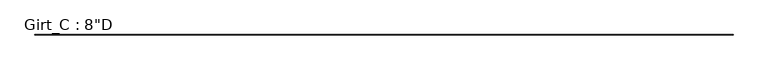
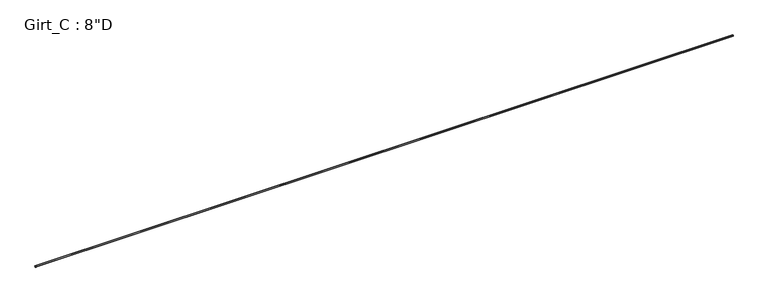
"""IFC4 building model written with IfcOpenShell, lengths in millimetres: beam geometry."""

from ifc_helpers import new_model, si_unit, point, frame, frame_2d, origin, place, context, project, spatial, polyline, circle_curve, trimmed, segment, composite_curve, outline, extrude, source, transform, mapped, element, save


def beam_86caec73(model_context):
    return source(origin(), model_context, "Body", "SweptSolid", [
        extrude(outline(composite_curve([segment(polyline([(63.5, 101.6), (75.745104, 87.0068534), (73.6169367, 85.221109), (62.204539, 98.821875), (3.3005807, 98.821875)]), True, "CONTINUOUS"), segment(trimmed(circle_curve(frame_2d((3.3741066, 96.8381931)), 1.9850441), [point((3.3005807, 98.821875))], [point((1.3890625, 96.8381931))], True, "CARTESIAN"), True, "CONTINUOUS"), segment(polyline([(1.3890625, 96.8381931), (1.3890625, -96.8389339)]), True, "CONTINUOUS"), segment(trimmed(circle_curve(frame_2d((3.3748024, -96.8389339)), 1.9857399), [point((1.3890625, -96.8389339))], [point((3.2694106, -98.821875))], True, "CARTESIAN"), True, "CONTINUOUS"), segment(polyline([(3.2694106, -98.821875), (62.204539, -98.821875), (73.6169367, -85.221109), (75.745104, -87.0068534), (63.5, -101.6), (3.3734375, -101.6)]), True, "CONTINUOUS"), segment(trimmed(circle_curve(frame_2d((3.3734375, -96.8375)), 4.7625), [point((3.3734375, -101.6))], [point((-1.3890625, -96.8375))], False, "CARTESIAN"), True, "CONTINUOUS"), segment(polyline([(-1.3890625, -96.8375), (-1.3890625, 96.8375)]), True, "CONTINUOUS"), segment(trimmed(circle_curve(frame_2d((3.3734375, 96.8375)), 4.7625), [point((-1.3890625, 96.8375))], [point((3.3734375, 101.6))], False, "CARTESIAN"), True, "CONTINUOUS"), segment(polyline([(3.3734375, 101.6), (63.5, 101.6)]), True, "CONTINUOUS")], self_intersect=False)), frame((-53222.525, 0.0, 0.0), z_axis=(1.0, 0.0, 0.0), x_axis=(0.0, 1.0, 0.0)), (0.0, 0.0, 1.0), 106445.05),
    ])


if __name__ == "__main__":
    model = new_model("IFC4")
    model_context = context("Model", 3, world=origin())
    ifc_project = project(units=[si_unit("LENGTHUNIT", "METRE", prefix="MILLI")], contexts=[model_context])
    site = spatial("IfcSite", under=ifc_project)
    building = spatial("IfcBuilding", under=site)
    placement = place(None, origin())
    beam_shape = beam_86caec73(model_context)
    element("IfcBeam", 1, ObjectType="Girt_C : 8\"D", at=placement, inside=building, context=model_context, shape_type="MappedRepresentation", body=[
        mapped(beam_shape, transform((0.0, 0.0, 0.0), x_axis=(1.0, 0.0, 0.0), y_axis=(0.0, 1.0, 0.0), z_axis=(0.0, 0.0, 1.0))),
    ])
    save(model, "model.ifc")

# Revit data of these elements
# Type "Girt_C : 8\"D"
#   Web_Thickness = 0' - 0 7/64"
#   Length [instance default] = 10' - 0"
#   Leg_1 = 0' - 2 1/2"
#   Height = 0' - 8"
#   Structural Material [instance default] = none
# Element 1 (IfcBeam, "Girt_C : 8\"D")
#   Structural Material = Steel
#   Materials on its faces: "Steel"
# Materials
#   "Steel": class "Metal", colour RGB 118 118 114, transparency 0, Description = "Steel, mill finish", Cost = 0
